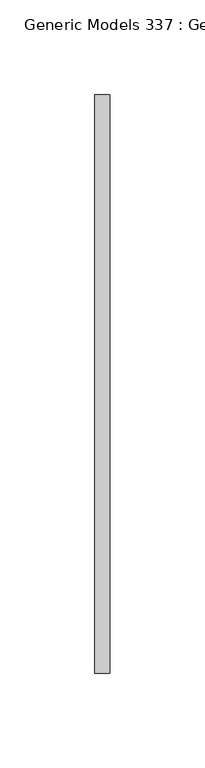
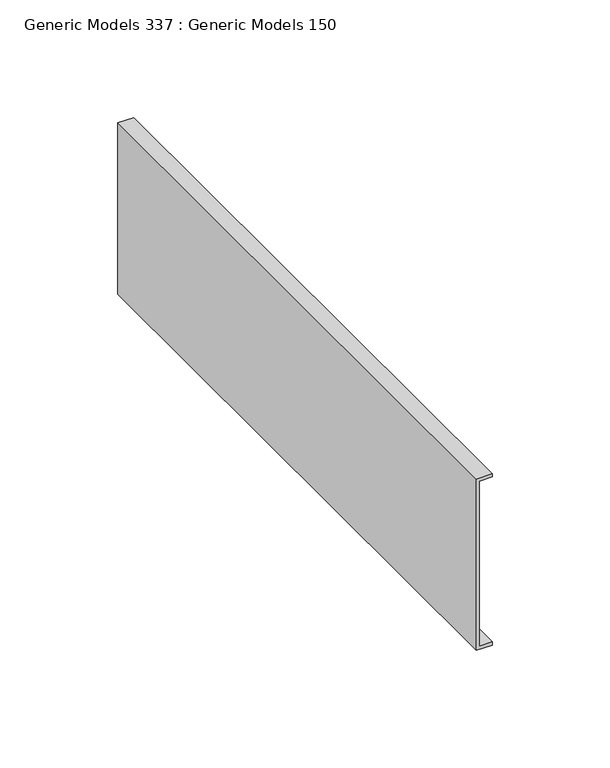
"""IFC4 building model written with IfcOpenShell, lengths in millimetres: proxy geometry, Generic Models 337 : Generic Models 150."""

import ifcopenshell
import ifcopenshell.guid

model = None  # the IFC model being written
_history = None  # IfcOwnerHistory: only IFC2X3 demands one
_inside = {}  # id of a spatial element -> (the spatial element, [elements in it])
_under = {}  # id of a project, library or spatial element -> (it, [spatial elements below it])
_declared = {}  # id of a project -> (the project, [libraries it declares])
_typed = {}  # id of a type object -> (the type object, [elements of that type])
_made_of = {}  # id of a material, layer set ... -> (it, [elements and type objects made of it])


def new_model(schema):
    """Start an empty IFC model of exactly this schema.

    Asked for "IFC4X3", IfcOpenShell would pick the latest addendum, in which some entities
    have other attributes; the version numbers below select the first issue.
    IFC2X3 requires an IfcOwnerHistory on every rooted entity: one is made here for all.
    """
    global model, _history
    if schema == "IFC4X3":
        model = ifcopenshell.file(schema_version=(4, 3, 0, 0))
    else:
        model = ifcopenshell.file(schema=schema)
    _inside.clear()
    _under.clear()
    _declared.clear()
    _typed.clear()
    _made_of.clear()
    _history = None
    if model.schema == "IFC2X3":
        org = make("IfcOrganization", Name="unknown")
        user = make(
            "IfcPersonAndOrganization",
            ThePerson=make("IfcPerson", FamilyName="unknown"),
            TheOrganization=org,
        )
        app = make(
            "IfcApplication",
            ApplicationDeveloper=org,
            Version="unknown",
            ApplicationFullName="unknown",
            ApplicationIdentifier="unknown",
        )
        _history = make(
            "IfcOwnerHistory",
            OwningUser=user,
            OwningApplication=app,
            ChangeAction="ADDED",
            CreationDate=0,
        )
    return model


def make(cls, **values):
    """One entity of the class cls with the attributes given. An attribute that is None is left unset."""
    return model.create_entity(
        cls, **{name: value for name, value in values.items() if value is not None}
    )


def rooted(cls, **values):
    """An entity with a GlobalId (a new one), such as an element, a storey or a relation."""
    return make(cls, GlobalId=ifcopenshell.guid.new(), OwnerHistory=_history, **values)


def si_unit(unit_type, name, prefix=None):
    """IfcSIUnit, for example si_unit("LENGTHUNIT", "METRE", prefix="MILLI")."""
    return make("IfcSIUnit", UnitType=unit_type, Prefix=prefix, Name=name)


def assignment(units):
    """IfcUnitAssignment: the units of a project."""
    return None if units is None else make("IfcUnitAssignment", Units=units)


def point(xyz):
    """IfcCartesianPoint."""
    return None if xyz is None else make("IfcCartesianPoint", Coordinates=xyz)


def direction(xyz):
    """IfcDirection."""
    return None if xyz is None else make("IfcDirection", DirectionRatios=xyz)


def frame(location, z_axis=None, x_axis=None):
    """IfcAxis2Placement3D, a coordinate frame: its origin and axes. An axis left out is left unset."""
    return make(
        "IfcAxis2Placement3D",
        Location=point(location),
        Axis=direction(z_axis),
        RefDirection=direction(x_axis),
    )


def origin():
    """The frame at (0, 0, 0) with its axes left unset."""
    return frame((0.0, 0.0, 0.0))


def place(relative_to, where):
    """IfcLocalPlacement: puts the frame where relative to a parent placement (None: the world)."""
    return make(
        "IfcLocalPlacement", PlacementRelTo=relative_to, RelativePlacement=where
    )


def context(
    kind, dimensions, precision=None, world=None, true_north=None, identifier=None
):
    """IfcGeometricRepresentationContext, for example the 3D "Model" context."""
    return make(
        "IfcGeometricRepresentationContext",
        ContextIdentifier=identifier,
        ContextType=kind,
        CoordinateSpaceDimension=dimensions,
        Precision=precision,
        WorldCoordinateSystem=world,
        TrueNorth=true_north,
    )


def project(units=None, contexts=None):
    """IfcProject with its units and contexts."""
    return rooted(
        "IfcProject",
        Name="project",
        RepresentationContexts=contexts,
        UnitsInContext=assignment(units),
    )


def spatial(cls, under=None, at=None, **own):
    """A site, building, storey or space (cls), placed at a placement, below another one or the project."""
    s = rooted(cls, ObjectPlacement=at, **own)
    if under is not None:
        _under.setdefault(under.id(), (under, []))[1].append(s)
    return s


def polyline(points):
    """IfcPolyline through the points."""
    return make("IfcPolyline", Points=[point(p) for p in points])


def outline(outer, holes=None, kind="AREA"):
    """IfcArbitraryClosedProfileDef: a profile drawn as a closed curve; with holes, ...WithVoids."""
    if holes is None:
        return make("IfcArbitraryClosedProfileDef", ProfileType=kind, OuterCurve=outer)
    return make(
        "IfcArbitraryProfileDefWithVoids",
        ProfileType=kind,
        OuterCurve=outer,
        InnerCurves=holes,
    )


def extrude(swept, where, along, depth):
    """IfcExtrudedAreaSolid: the profile swept, set in the frame where, extruded along a direction by depth."""
    return make(
        "IfcExtrudedAreaSolid",
        SweptArea=swept,
        Position=where,
        ExtrudedDirection=direction(along),
        Depth=depth,
    )


def shape(context_of_items, identifier, shape_type, items):
    """IfcShapeRepresentation: the items that make up one representation, for example the "Body"."""
    return make(
        "IfcShapeRepresentation",
        ContextOfItems=context_of_items,
        RepresentationIdentifier=identifier,
        RepresentationType=shape_type,
        Items=items,
    )


def source(mapping_origin, context_of_items, identifier, shape_type, items):
    """IfcRepresentationMap: a shape defined once, which mapped items show again and again."""
    return make(
        "IfcRepresentationMap",
        MappingOrigin=mapping_origin,
        MappedRepresentation=shape(context_of_items, identifier, shape_type, items),
    )


def transform(
    local_origin,
    x_axis=None,
    y_axis=None,
    z_axis=None,
    scale=None,
    scale2=None,
    scale3=None,
    uniform=True,
):
    """IfcCartesianTransformationOperator3D, or its non-uniform kind. x_axis, y_axis, z_axis: its Axis1, 2, 3."""
    if uniform:
        return make(
            "IfcCartesianTransformationOperator3D",
            Axis1=direction(x_axis),
            Axis2=direction(y_axis),
            LocalOrigin=point(local_origin),
            Scale=scale,
            Axis3=direction(z_axis),
        )
    return make(
        "IfcCartesianTransformationOperator3DnonUniform",
        Axis1=direction(x_axis),
        Axis2=direction(y_axis),
        LocalOrigin=point(local_origin),
        Scale=scale,
        Axis3=direction(z_axis),
        Scale2=scale2,
        Scale3=scale3,
    )


def mapped(mapping_source, mapping_target):
    """IfcMappedItem: shows the shape of a source again, moved by a transform."""
    return make(
        "IfcMappedItem", MappingSource=mapping_source, MappingTarget=mapping_target
    )


def made_of(thing, what):
    """Note that an element or type object is made of a material, layer set ...; save() writes the relation."""
    if what is not None:
        _made_of.setdefault(what.id(), (what, []))[1].append(thing)
    return thing


def element(
    cls,
    number,
    at=None,
    inside=None,
    cuts=None,
    type_object=None,
    material=None,
    context=None,
    identifier="Body",
    shape_type=None,
    held_by="IfcProductDefinitionShape",
    body=None,
    shapes=None,
    **own,
):
    """One element of the class cls, such as IfcWall. Its Tag is "e" and its number.

    at: its placement. inside: the storey or other place that contains it. cuts: it is an
    opening in that element (IfcRelVoidsElement). A single representation is given by context,
    identifier, shape_type and body (its items); several are given by shapes. held_by: the class
    of the entity that holds the representations. save() writes the other relations.
    """
    e = rooted(cls, Tag="e%d" % number, ObjectPlacement=at, **own)
    if body is not None:
        shapes = [shape(context, identifier, shape_type, body)]
    if shapes is not None:
        e.Representation = make(held_by, Representations=shapes)
    if inside is not None:
        _inside.setdefault(inside.id(), (inside, []))[1].append(e)
    if cuts is not None:
        rooted(
            "IfcRelVoidsElement", RelatingBuildingElement=cuts, RelatedOpeningElement=e
        )
    if type_object is not None:
        _typed.setdefault(type_object.id(), (type_object, []))[1].append(e)
    return made_of(e, material)


def aggregate(whole, parts):
    """IfcRelAggregates: a whole, such as a stair, and the parts it consists of."""
    return rooted("IfcRelAggregates", RelatingObject=whole, RelatedObjects=parts)


def save(model, path):
    """Write the relations noted so far, then the file.

    IfcRelAggregates (storeys below a building ...), IfcRelContainedInSpatialStructure (elements
    in a storey), IfcRelDefinesByType, IfcRelAssociatesMaterial and IfcRelDeclares: one each for
    every whole, place, type object, material and project.
    """
    for whole, parts in _under.values():
        aggregate(whole, parts)
    for where, things in _inside.values():
        rooted(
            "IfcRelContainedInSpatialStructure",
            RelatedElements=things,
            RelatingStructure=where,
        )
    for kind, things in _typed.values():
        rooted("IfcRelDefinesByType", RelatedObjects=things, RelatingType=kind)
    for what, things in _made_of.values():
        rooted("IfcRelAssociatesMaterial", RelatedObjects=things, RelatingMaterial=what)
    for by, libraries in _declared.values():
        rooted("IfcRelDeclares", RelatingContext=by, RelatedDefinitions=libraries)
    model.write(path)


def generic_models_337_generic_models_150_18aad3a8(model_context):
    return source(origin(), model_context, "Body", "SweptSolid", [
        extrude(outline(polyline([(126274.2676453, 4830.1377227), (126274.2676453, 4836.4877227), (126275.8551453, 4836.4877227), (126275.8551453, 4828.5502227), (126186.9837007, 4828.5502227), (126186.9837007, 4836.4877227), (126188.5712007, 4836.4877227), (126188.5712007, 4830.1377227), (126274.2676453, 4830.1377227)])), frame((0.0, 399.7309662, 0.0), z_axis=(0.0, 1.0, 0.0), x_axis=(0.0, 0.0, 1.0)), (0.0, 0.0, 1.0), 304.8),
    ])


if __name__ == "__main__":
    model = new_model("IFC4")
    model_context = context("Model", 3, world=origin())
    ifc_project = project(units=[si_unit("LENGTHUNIT", "METRE", prefix="MILLI")], contexts=[model_context])
    site = spatial("IfcSite", under=ifc_project)
    building = spatial("IfcBuilding", under=site)
    placement = place(None, origin())
    generic_models_337_generic_models_150_shape = generic_models_337_generic_models_150_18aad3a8(model_context)
    element("IfcBuildingElementProxy", 1, Name="Generic Models 337 : Generic Models 150", ObjectType="Generic Models 337 : Generic Models 150", at=placement, inside=building, context=model_context, shape_type="MappedRepresentation", body=[
        mapped(generic_models_337_generic_models_150_shape, transform((0.0, 0.0, 0.0), x_axis=(1.0, 0.0, 0.0), y_axis=(0.0, 1.0, 0.0), z_axis=(0.0, 0.0, 1.0))),
    ])
    save(model, "model.ifc")

# Revit data of these elements
# Element 1 (IfcBuildingElementProxy, "Generic Models 337 : Generic Models 150")
#   Materials on its faces: "_ALUM. MULLION CAP BY WINDOW MANUFACTURER (COLOR T.B.D)"
# Materials
#   "_ALUM. MULLION CAP BY WINDOW MANUFACTURER (COLOR T.B.D)": class "Metal", colour RGB 199 199 199, transparency 0, Description = "Structural steel 50ksi", Cost = 0
